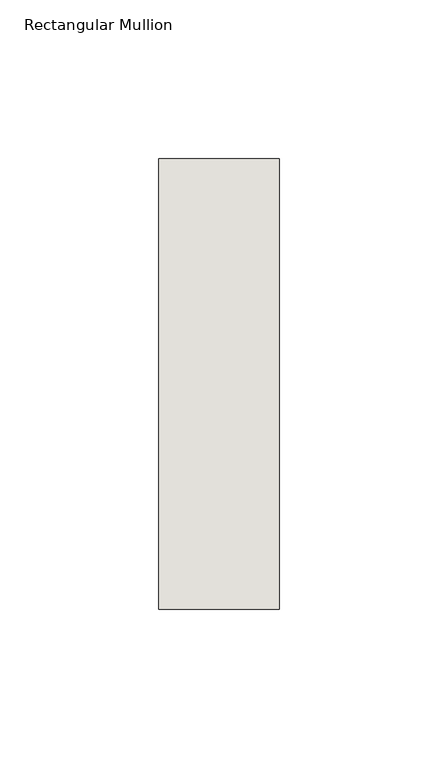
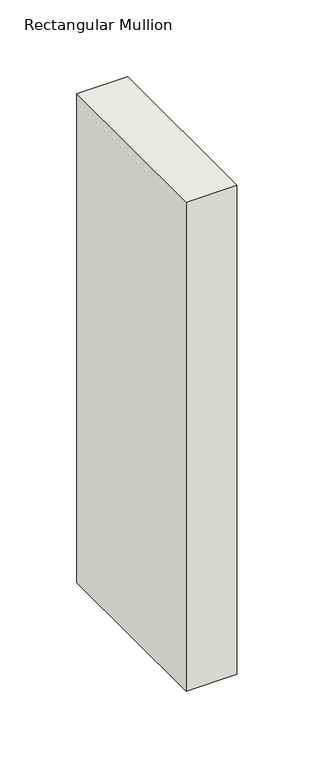
"""IFC4 building model written with IfcOpenShell, lengths in millimetres: wall geometry, Rectangular Mullion : NLRS_21_CWM_hsb-regel 38x142_gen_rsf."""

from ifc_helpers import new_model, si_unit, frame, origin, place, context, project, spatial, polyline, outline, extrude, source, transform, mapped, element, save


def rectangular_mullion_05042751(model_context):
    return source(origin(), model_context, "Body", "SweptSolid", [
        extrude(outline(polyline([(19.0, -71.0), (-19.0, -71.0), (-19.0, 71.0), (19.0, 71.0), (19.0, -71.0)])), frame((0.0, 0.0, -388.0), z_axis=(0.0, 0.0, 1.0), x_axis=(1.0, 0.0, 0.0)), (0.0, 0.0, 1.0), 388.0),
    ])


if __name__ == "__main__":
    model = new_model("IFC4")
    model_context = context("Model", 3, world=origin())
    ifc_project = project(units=[si_unit("LENGTHUNIT", "METRE", prefix="MILLI")], contexts=[model_context])
    site = spatial("IfcSite", under=ifc_project)
    building = spatial("IfcBuilding", under=site)
    placement = place(None, origin())
    rectangular_mullion_shape = rectangular_mullion_05042751(model_context)
    element("IfcWall", 1, ObjectType="Rectangular Mullion : NLRS_21_CWM_hsb-regel 38x142_gen_rsf", at=placement, inside=building, context=model_context, shape_type="MappedRepresentation", body=[
        mapped(rectangular_mullion_shape, transform((0.0, 0.0, 0.0), x_axis=(1.0, 0.0, 0.0), y_axis=(0.0, 1.0, 0.0), z_axis=(0.0, 0.0, 1.0))),
    ])
    save(model, "model.ifc")

# Revit data of these elements
# Type "Rectangular Mullion : NLRS_21_CWM_hsb-regel 38x142_gen_rsf"
#   Type IfcGUID = "07M7mRoiH1CR8m_RSKIwpF"
#   Assembly Code = "21.10"
#   IfcExportAs = "IfcWall"
#   built-in parameter 1007322 = 0.465879 (stored number, unit not read)
#   built-in parameter 1007321 = 0.062336 (stored number, unit not read)
#   built-in parameter 1007320 = 0.062336 (stored number, unit not read)
# Element 1 (IfcWall, "Rectangular Mullion : NLRS_21_CWM_hsb-regel 38x142_gen_rsf")
#   Materials on its faces: "NLRS_i2_hout naaldhout vuren_gen_rsf"
# Materials
#   "NLRS_i2_hout naaldhout vuren_gen_rsf": class "I - Hout", colour RGB 234 199 147, transparency 0, Keynote = "i2", Manufacturer = "Revit Standards Foundation", URL = "www.revitstandards.org", Description = "hout vuren", Cost = 0
